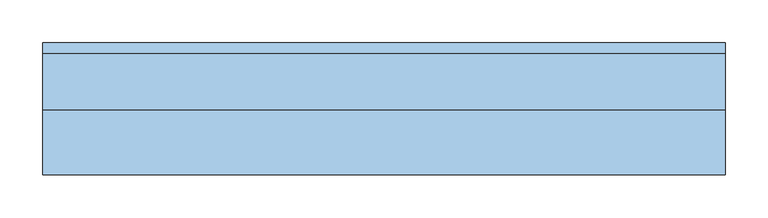
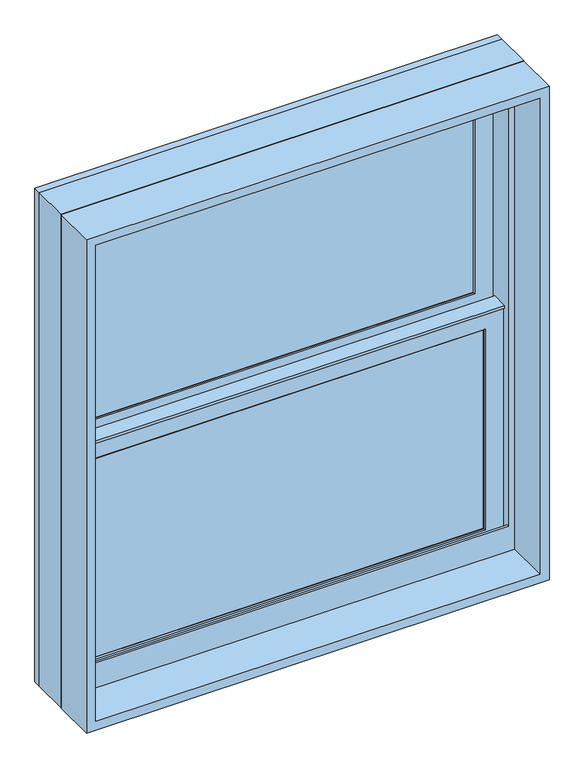
"""IFC4 building model written with IfcOpenShell, lengths in millimetres: window geometry, Window-Double_Hung-Marvin-Essential : ESDH2830."""

from ifc_helpers import new_model, si_unit, frame, origin, place, context, project, spatial, polyline, outline, extrude, faceted_brep, source, transform, mapped, element, save


def window_2e39aaf6(model_context):
    return source(origin(), model_context, "Body", "SolidModel", [
        extrude(outline(polyline([(123.825, 20.6375), (123.825, 15.875), (104.775, 15.875), (104.775, 20.6375), (123.825, 20.6375)])), frame((0.0, 0.0, 1593.85), z_axis=(0.0, 0.0, 1.0), x_axis=(1.0, 0.0, 0.0)), (0.0, 0.0, 1.0), 374.65),
        extrude(outline(polyline([(-104.775, 20.6375), (-104.775, 15.875), (-123.825, 15.875), (-123.825, 20.6375), (-104.775, 20.6375)])), frame((0.0, 0.0, 1593.85), z_axis=(0.0, 0.0, 1.0), x_axis=(1.0, 0.0, 0.0)), (0.0, 0.0, 1.0), 374.65),
        extrude(outline(polyline([(342.9, 20.6375), (342.9, 15.875), (-342.9, 15.875), (-342.9, 20.6375), (342.9, 20.6375)])), frame((0.0, 0.0, 1771.65), z_axis=(0.0, 0.0, 1.0), x_axis=(1.0, 0.0, 0.0)), (0.0, 0.0, 1.0), 19.05),
        extrude(outline(polyline([(-123.825, 46.83125), (-123.825, 51.59375), (-104.775, 51.59375), (-104.775, 46.83125), (-123.825, 46.83125)])), frame((0.0, 0.0, 2006.6), z_axis=(0.0, 0.0, 1.0), x_axis=(1.0, 0.0, 0.0)), (0.0, 0.0, 1.0), 374.65),
        extrude(outline(polyline([(104.775, 46.83125), (104.775, 51.59375), (123.825, 51.59375), (123.825, 46.83125), (104.775, 46.83125)])), frame((0.0, 0.0, 2006.6), z_axis=(0.0, 0.0, 1.0), x_axis=(1.0, 0.0, 0.0)), (0.0, 0.0, 1.0), 374.65),
        extrude(outline(polyline([(-342.9, 46.83125), (-342.9, 51.59375), (342.9, 51.59375), (342.9, 46.83125), (-342.9, 46.83125)])), frame((0.0, 0.0, 2184.4), z_axis=(0.0, 0.0, 1.0), x_axis=(1.0, 0.0, 0.0)), (0.0, 0.0, 1.0), 19.05),
        extrude(outline(polyline([(123.825, 20.6375), (104.775, 20.6375), (104.775, 25.4), (123.825, 25.4), (123.825, 20.6375)])), frame((0.0, 0.0, 1593.85), z_axis=(0.0, 0.0, 1.0), x_axis=(1.0, 0.0, 0.0)), (0.0, 0.0, 1.0), 374.65),
        extrude(outline(polyline([(-104.775, 20.6375), (-123.825, 20.6375), (-123.825, 25.4), (-104.775, 25.4), (-104.775, 20.6375)])), frame((0.0, 0.0, 1593.85), z_axis=(0.0, 0.0, 1.0), x_axis=(1.0, 0.0, 0.0)), (0.0, 0.0, 1.0), 374.65),
        extrude(outline(polyline([(342.9, 20.6375), (-342.9, 20.6375), (-342.9, 25.4), (342.9, 25.4), (342.9, 20.6375)])), frame((0.0, 0.0, 1771.65), z_axis=(0.0, 0.0, 1.0), x_axis=(1.0, 0.0, 0.0)), (0.0, 0.0, 1.0), 19.05),
        extrude(outline(polyline([(-123.825, 56.35625), (-104.775, 56.35625), (-104.775, 51.59375), (-123.825, 51.59375), (-123.825, 56.35625)])), frame((0.0, 0.0, 2006.6), z_axis=(0.0, 0.0, 1.0), x_axis=(1.0, 0.0, 0.0)), (0.0, 0.0, 1.0), 374.65),
        extrude(outline(polyline([(104.775, 56.35625), (123.825, 56.35625), (123.825, 51.59375), (104.775, 51.59375), (104.775, 56.35625)])), frame((0.0, 0.0, 2006.6), z_axis=(0.0, 0.0, 1.0), x_axis=(1.0, 0.0, 0.0)), (0.0, 0.0, 1.0), 374.65),
        extrude(outline(polyline([(-342.9, 56.35625), (342.9, 56.35625), (342.9, 51.59375), (-342.9, 51.59375), (-342.9, 56.35625)])), frame((0.0, 0.0, 2184.4), z_axis=(0.0, 0.0, 1.0), x_axis=(1.0, 0.0, 0.0)), (0.0, 0.0, 1.0), 19.05),
        faceted_brep([(-369.8875, 5.6780605, 1998.5351748), (-369.8875, 5.6780605, 1993.9), (369.8875, 5.6780605, 1993.9), (369.8875, 5.6780605, 1998.5351748), (-369.8875, 34.8118605, 1998.5351748), (369.8875, 34.8118605, 1998.5351748), (369.8875, 34.8118605, 1993.9), (-369.8875, 34.8118605, 1993.9), (-369.8875, 30.1625, 1993.9), (-369.8875, 30.1625, 1566.8625), (-369.8875, 8.9241104, 1566.8625), (-369.8875, 8.9241104, 1993.9), (369.8875, 8.9241104, 1993.9), (369.8875, 30.1625, 1993.9), (369.8875, 8.9241104, 1566.8625), (369.8875, 30.1625, 1566.8625), (-354.0034752, 11.90625, 1979.6034752), (-354.0034752, 30.1625, 1979.6034752), (354.0034752, 30.1625, 1979.6034752), (354.0034752, 11.90625, 1979.6034752), (-337.34375, 10.4662439, 1962.94375), (-337.34375, 11.90625, 1962.94375), (337.34375, 11.90625, 1962.94375), (337.34375, 10.4662439, 1962.94375), (338.8858834, 8.9241104, 1964.4858834), (-338.8858834, 8.9241104, 1964.4858834), (354.0034752, 30.1625, 1582.7465248), (354.0034752, 11.90625, 1582.7465248), (337.34375, 11.90625, 1599.40625), (337.34375, 10.4662439, 1599.40625), (338.8858834, 8.9241104, 1597.8641166), (-354.0034752, 30.1625, 1582.7465248), (-354.0034752, 11.90625, 1582.7465248), (-337.34375, 11.90625, 1599.40625), (-337.34375, 10.4662439, 1599.40625), (-338.8858834, 8.9241104, 1597.8641166)], [[[0, 1, 2, 3]], [[4, 5, 6, 7]], [[1, 0, 4, 7, 8, 9, 10, 11]], [[2, 1, 11, 12]], [[7, 6, 13, 8]], [[3, 2, 12, 14, 15, 13, 6, 5]], [[0, 3, 5, 4]], [[16, 17, 18, 19]], [[20, 21, 22, 23]], [[20, 23, 24, 25]], [[19, 18, 26, 27]], [[23, 22, 28, 29]], [[24, 23, 29, 30]], [[27, 26, 31, 32]], [[29, 28, 33, 34]], [[30, 29, 34, 35]], [[15, 14, 10, 9]], [[15, 9, 8, 13], [18, 17, 31, 26]], [[17, 16, 32, 31]], [[16, 19, 27, 32], [22, 21, 33, 28]], [[21, 20, 34, 33]], [[20, 25, 35, 34]], [[10, 14, 12, 11], [25, 24, 30, 35]]]),
        extrude(outline(polyline([(38.5955581, 1979.6125), (33.5778968, 1979.6125), (33.5778968, 1981.2), (39.9405976, 1981.2), (39.9405976, 1979.6125), (61.515625, 1979.6125), (47.6307501, 1976.2975159), (38.5955581, 1976.2975159), (38.5955581, 1979.6125)])), frame((-369.8875, 0.0, 0.0), z_axis=(1.0, 0.0, 0.0), x_axis=(0.0, 1.0, 0.0)), (0.0, 0.0, 1.0), 739.775),
        faceted_brep([(400.05, 0.0, 1536.7), (400.05, 0.0, 2438.4), (-400.05, 0.0, 2438.4), (-400.05, 0.0, 1536.7), (373.85625, 0.0, 1597.81875), (-373.85625, 0.0, 1597.81875), (-373.85625, 0.0, 2412.20625), (373.85625, 0.0, 2412.20625), (373.85625, 3.96875, 1536.7), (-373.85625, 3.96875, 1536.7), (-373.85625, 3.96875, 1597.81875), (373.85625, 3.96875, 1597.81875), (-400.05, 65.6828125, 1536.7), (-373.85625, 65.6828125, 1536.7), (373.85625, 65.6828125, 1536.7), (400.05, 65.6828125, 1536.7), (-400.05, 65.6828125, 2438.4), (400.05, 65.6828125, 2438.4), (373.85625, 65.6828125, 2412.20625), (-373.85625, 65.6828125, 2412.20625)], [[[0, 1, 2, 3], [4, 5, 6, 7]], [[8, 9, 10, 11]], [[5, 4, 11, 10]], [[0, 3, 12, 13, 9, 8, 14, 15]], [[13, 12, 16, 17, 15, 14, 18, 19]], [[13, 19, 6, 5, 10, 9]], [[7, 6, 19, 18]], [[18, 14, 8, 11, 4, 7]], [[1, 0, 15, 17]], [[2, 1, 17, 16]], [[3, 2, 16, 12]]]),
        faceted_brep([(373.85625, 30.1625, 1987.55), (372.26875, 30.1625, 1987.55), (372.26875, 30.1625, 1561.0544613), (373.85625, 30.1625, 1561.0544613), (-372.26875, 30.1625, 1987.55), (-373.85625, 30.1625, 1987.55), (-373.85625, 30.1625, 1561.0544613), (-372.26875, 30.1625, 1561.0544613), (372.26875, 63.5, 1987.55), (373.85625, 63.5, 1987.55), (373.85625, 63.5, 1554.5743077), (372.26875, 63.5, 1554.5743077), (-373.85625, 63.5, 1987.55), (-372.26875, 63.5, 1987.55), (-372.26875, 63.5, 1554.5743077), (-373.85625, 63.5, 1554.5743077), (385.1108932, 3.96875, 1566.1460105), (385.1108932, 3.96875, 1536.7), (385.1108932, 65.6828125, 1536.7), (385.1108932, 65.6828125, 1554.150012), (-385.1108932, 3.96875, 1536.7), (-385.1108932, 3.96875, 1566.1460105), (-385.1108932, 65.6828125, 1554.150012), (-385.1108932, 65.6828125, 1536.7), (385.1108932, 78.58125, 1551.6428097), (-385.1108932, 78.58125, 1551.6428097), (-383.0971252, 68.2348864, 1553.6539391), (-365.13135, 68.2348864, 1553.6539391), (-365.13135, 65.6828125, 1554.150012), (365.13135, 65.6828125, 1554.150012), (365.13135, 68.2348864, 1553.6539391), (383.0971252, 68.2348864, 1553.6539391), (-400.05, 65.6828125, 1536.7), (-400.05, 78.5948249, 1536.7), (400.05, 78.5948249, 1536.7), (400.05, 65.6828125, 1536.7), (-400.05, 78.58125, 2438.4), (400.05, 78.58125, 2438.4), (385.1108932, 78.58125, 2423.4608932), (-385.1108932, 78.58125, 2423.4608932), (-400.05, 65.6828125, 2438.4), (-383.0971252, 68.2348864, 2421.4471252), (383.0971252, 68.2348864, 2421.4471252), (365.13135, 68.2348864, 2403.48135), (-365.13135, 68.2348864, 2403.48135), (-365.13135, 65.6828125, 2403.48135), (365.13135, 65.6828125, 2403.48135), (400.05, 65.6828125, 2438.4)], [[[0, 1, 2, 3]], [[4, 5, 6, 7]], [[8, 9, 10, 11]], [[12, 13, 14, 15]], [[1, 8, 11, 2]], [[9, 0, 3, 10]], [[1, 0, 9, 8]], [[5, 4, 13, 12]], [[5, 12, 15, 6]], [[13, 4, 7, 14]], [[16, 17, 18, 19]], [[20, 21, 22, 23]], [[24, 25, 26, 27, 28, 22, 21, 16, 19, 29, 30, 31], [3, 2, 11, 10], [7, 6, 15, 14]], [[17, 16, 21, 20]], [[17, 20, 23, 32, 33, 34, 35, 18]], [[34, 33, 36, 37], [25, 24, 38, 39]], [[33, 32, 40, 36]], [[39, 41, 26, 25]], [[41, 42, 31, 30, 43, 44, 27, 26]], [[44, 45, 28, 27]], [[40, 32, 23, 22, 28, 45, 46, 29, 19, 18, 35, 47]], [[36, 40, 47, 37]], [[39, 38, 42, 41]], [[44, 43, 46, 45]], [[34, 37, 47, 35]], [[42, 38, 24, 31]], [[46, 43, 30, 29]]]),
        extrude(outline(polyline([(350.04375, 11.90625), (-350.04375, 11.90625), (-350.04375, 15.08125), (350.04375, 15.08125), (350.04375, 11.90625)])), frame((0.0, 0.0, 1586.70625), z_axis=(0.0, 0.0, 1.0), x_axis=(1.0, 0.0, 0.0)), (0.0, 0.0, 1.0), 388.9375),
        extrude(outline(polyline([(350.04375, 42.8625), (-350.04375, 42.8625), (-350.04375, 46.0375), (350.04375, 46.0375), (350.04375, 42.8625)])), frame((0.0, 0.0, 1999.45625), z_axis=(0.0, 0.0, 1.0), x_axis=(1.0, 0.0, 0.0)), (0.0, 0.0, 1.0), 388.9375),
        faceted_brep([(-337.34375, 31.194477, 1962.94375), (-338.8858834, 32.7366104, 1964.4858834), (338.8858834, 32.7366104, 1964.4858834), (337.34375, 31.194477, 1962.94375), (-337.34375, 30.1625, 1962.94375), (337.34375, 30.1625, 1962.94375), (-369.8875, 32.7366104, 1995.4875), (-369.8875, 30.1625, 1995.4875), (369.8875, 30.1625, 1995.4875), (369.8875, 32.7366104, 1995.4875), (338.8858834, 32.7366104, 1597.8641166), (337.34375, 31.194477, 1599.40625), (337.34375, 30.1625, 1599.40625), (369.8875, 30.1625, 1566.8625), (369.8875, 32.7366104, 1566.8625), (-338.8858834, 32.7366104, 1597.8641166), (-337.34375, 31.194477, 1599.40625), (-337.34375, 30.1625, 1599.40625), (-369.8875, 30.1625, 1566.8625), (-369.8875, 32.7366104, 1566.8625)], [[[0, 1, 2, 3]], [[4, 0, 3, 5]], [[6, 7, 8, 9]], [[3, 2, 10, 11]], [[5, 3, 11, 12]], [[9, 8, 13, 14]], [[11, 10, 15, 16]], [[12, 11, 16, 17]], [[14, 13, 18, 19]], [[9, 14, 19, 6], [1, 15, 10, 2]], [[16, 15, 1, 0]], [[17, 16, 0, 4]], [[7, 18, 13, 8], [5, 12, 17, 4]], [[19, 18, 7, 6]]]),
        faceted_brep([(-354.0034752, 42.8625, 2392.3534752), (-354.0034752, 61.11875, 2392.3534752), (354.0034752, 61.11875, 2392.3534752), (354.0034752, 42.8625, 2392.3534752), (-337.34375, 41.4224939, 2375.69375), (-337.34375, 42.8625, 2375.69375), (337.34375, 42.8625, 2375.69375), (337.34375, 41.4224939, 2375.69375), (-338.8858834, 39.8803604, 2377.2358834), (338.8858834, 39.8803604, 2377.2358834), (-369.8875, 61.11875, 2408.2375), (-369.8875, 39.8803604, 2408.2375), (369.8875, 39.8803604, 2408.2375), (369.8875, 61.11875, 2408.2375), (354.0034752, 61.11875, 1995.4965248), (354.0034752, 42.8625, 1995.4965248), (337.34375, 42.8625, 2012.15625), (337.34375, 41.4224939, 2012.15625), (338.8858834, 39.8803604, 2010.6141166), (369.8875, 39.8803604, 1979.6125), (369.8875, 61.11875, 1979.6125), (-354.0034752, 61.11875, 1995.4965248), (-354.0034752, 42.8625, 1995.4965248), (-337.34375, 42.8625, 2012.15625), (-337.34375, 41.4224939, 2012.15625), (-338.8858834, 39.8803604, 2010.6141166), (-369.8875, 39.8803604, 1979.6125), (-369.8875, 61.11875, 1979.6125)], [[[0, 1, 2, 3]], [[4, 5, 6, 7]], [[8, 4, 7, 9]], [[10, 11, 12, 13]], [[3, 2, 14, 15]], [[7, 6, 16, 17]], [[9, 7, 17, 18]], [[13, 12, 19, 20]], [[15, 14, 21, 22]], [[17, 16, 23, 24]], [[18, 17, 24, 25]], [[20, 19, 26, 27]], [[13, 20, 27, 10], [1, 21, 14, 2]], [[22, 21, 1, 0]], [[3, 15, 22, 0], [5, 23, 16, 6]], [[24, 23, 5, 4]], [[25, 24, 4, 8]], [[11, 26, 19, 12], [9, 18, 25, 8]], [[27, 26, 11, 10]]]),
        faceted_brep([(-369.8875, 61.11875, 1979.6125), (-369.8875, 63.6928604, 1979.6125), (369.8875, 63.6928604, 1979.6125), (369.8875, 61.11875, 1979.6125), (-337.34375, 62.150727, 2012.15625), (-337.34375, 61.11875, 2012.15625), (337.34375, 61.11875, 2012.15625), (337.34375, 62.150727, 2012.15625), (-338.8858834, 63.6928604, 2010.6141166), (338.8858834, 63.6928604, 2010.6141166), (369.8875, 63.6928604, 2408.2375), (369.8875, 61.11875, 2408.2375), (337.34375, 61.11875, 2375.69375), (337.34375, 62.150727, 2375.69375), (338.8858834, 63.6928604, 2377.2358834), (-369.8875, 63.6928604, 2408.2375), (-369.8875, 61.11875, 2408.2375), (-337.34375, 61.11875, 2375.69375), (-337.34375, 62.150727, 2375.69375), (-338.8858834, 63.6928604, 2377.2358834)], [[[0, 1, 2, 3]], [[4, 5, 6, 7]], [[8, 4, 7, 9]], [[3, 2, 10, 11]], [[7, 6, 12, 13]], [[9, 7, 13, 14]], [[11, 10, 15, 16]], [[13, 12, 17, 18]], [[14, 13, 18, 19]], [[16, 15, 1, 0]], [[3, 11, 16, 0], [5, 17, 12, 6]], [[18, 17, 5, 4]], [[19, 18, 4, 8]], [[1, 15, 10, 2], [9, 14, 19, 8]]]),
        extrude(outline(polyline([(350.04375, 26.19375), (-350.04375, 26.19375), (-350.04375, 30.1625), (350.04375, 30.1625), (350.04375, 26.19375)])), frame((0.0, 0.0, 1586.70625), z_axis=(0.0, 0.0, 1.0), x_axis=(1.0, 0.0, 0.0)), (0.0, 0.0, 1.0), 388.9375),
        extrude(outline(polyline([(350.04375, 57.15), (-350.04375, 57.15), (-350.04375, 61.11875), (350.04375, 61.11875), (350.04375, 57.15)])), frame((0.0, 0.0, 1999.45625), z_axis=(0.0, 0.0, 1.0), x_axis=(1.0, 0.0, 0.0)), (0.0, 0.0, 1.0), 388.9375),
        extrude(outline(polyline([(2438.4, 400.05), (2438.4, -400.05), (1536.7, -400.05), (1536.7, 400.05), (2438.4, 400.05)]), holes=[polyline([(2422.525, 384.175), (1552.575, 384.175), (1552.575, -384.175), (2422.525, -384.175), (2422.525, 384.175)])]), frame((0.0, -76.2, 0.0), z_axis=(0.0, 1.0, 0.0), x_axis=(0.0, 0.0, 1.0)), (0.0, 0.0, 1.0), 75.40625),
    ])


if __name__ == "__main__":
    model = new_model("IFC4")
    model_context = context("Model", 3, world=origin())
    ifc_project = project(units=[si_unit("LENGTHUNIT", "METRE", prefix="MILLI")], contexts=[model_context])
    site = spatial("IfcSite", under=ifc_project)
    building = spatial("IfcBuilding", under=site)
    placement = place(None, origin())
    window_shape = window_2e39aaf6(model_context)
    element("IfcWindow", 1, ObjectType="Window-Double_Hung-Marvin-Essential : ESDH2830", at=placement, inside=building, context=model_context, shape_type="MappedRepresentation", body=[
        mapped(window_shape, transform((0.0, 0.0, 0.0), x_axis=(1.0, 0.0, 0.0), y_axis=(0.0, 1.0, 0.0), z_axis=(0.0, 0.0, 1.0))),
    ])
    save(model, "model.ifc")

# Revit data of these elements
# Type "Window-Double_Hung-Marvin-Essential : ESDH2830"
#   Type Mark = "36"
#   Window Type = "Essential Double Hung"
#   Product data url = "https://bimobject.com/marvin-windows-and-doors/product/marvin-dhwau"
#   Product Guid = "c4a96547-874c-4385-91dc-a058adc19d98"
#   Frame = "All Ultrex"
#   Egress Window = "No"
#   URL = "www.marvin.com"
#   Model = "ESDH2830"
#   Manufacturer = "Marvin Windows and Doors"
#   Label Egress = ""
#   Glass Type = "IG Low E II with Argon"
#   Design Pressure = "DP50"
#   Description = "3236 DBHG"
#   Analytic Construction = "<None>"
#   Prairie Corner Width = 0' - 4"
#   Prairie Corner Height = 0' - 4"
#   Egress Width = 2' - 4 9/16"
#   Egress Height = 1' - 1 27/128"
#   Rough Width = 2' - 8"
#   Rough Height = 3' - 0"
#   Nominal Width = 2' - 8"
#   Nominal Height = 3' - 0"
#   Inset to Installation Flange [instance default] = 0' - 1"
#   Height = 2' - 11 1/2"
#   Egress Area = 2.6204 SF
#   Default Head Height = 8' - 0"
#   Width = 2' - 7 1/2"
#   Daylight Area = 5.28022 SF
#   DLO Width = 2' - 2 9/16"
#   DLO Height = 1' - 2 5/16"
#   Muntins Top Sash = yes
#   Lites Wide Top Sash = 3
#   Lites Wide Bottom Sash = 3
#   Lites High Top Sash = 2
#   Lites High Bottom Sash = 2
#   Lite Cut Prairie 9 = no
#   Lite Cut HV Grid = yes
#   Muntins Bottom Sash = yes
#   Label Visibility = no
#   Jamb Extension Visibility = yes
#   Edition number = 1
#   Interior Material = Ultrex-Marvin-Stonewhite
#   Glazing Material = Glass-Marvin-IG Low E II with Argon
#   Cladding Material = Ultrex-Marvin-Pebblegray
#   Wall Closure = (empty or 0)
#   Assembly Code = ""
# Element 1 (IfcWindow, "Window-Double_Hung-Marvin-Essential : ESDH2830")
#   Materials on its faces: "Ultrex-Marvin-Pebblegray", "Ultrex-Marvin-Stonewhite", "Glass-Marvin-IG Low E II with Argon"
# Materials
#   "Ultrex-Marvin-Stonewhite": class "Paint", colour RGB 250 251 245, transparency 0
#   "Glass-Marvin-IG Low E II with Argon": class "Glass", colour RGB 0 128 192, transparency 0.85
#   "Ultrex-Marvin-Pebblegray": class "Paint", colour RGB 189 185 173, transparency 0
